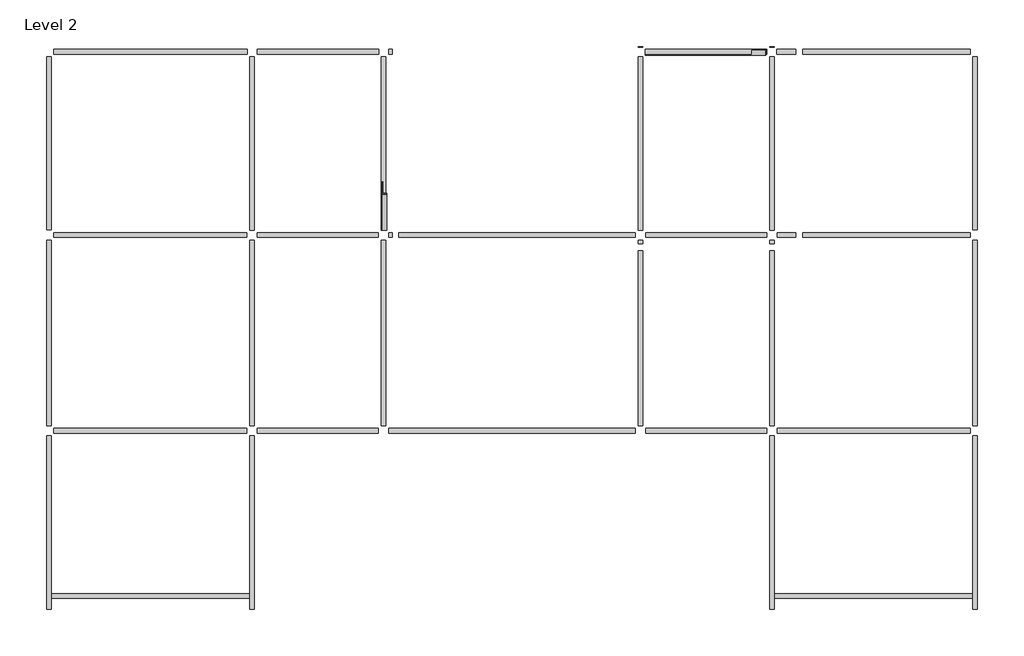
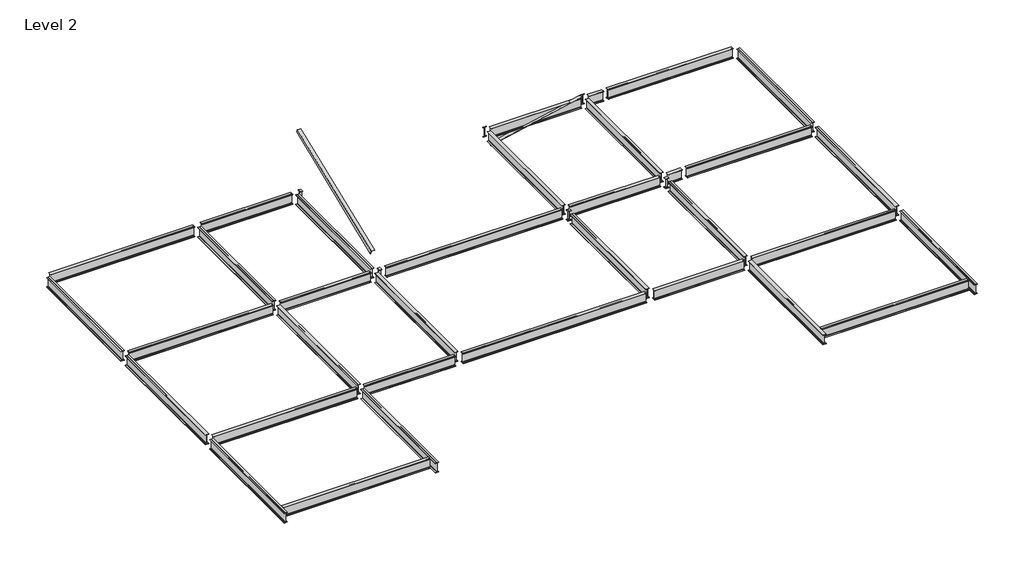
# One storey: 40 beams, 2 members.
"""IFC4 building model written with IfcOpenShell, lengths in millimetres."""

import ifcopenshell
import ifcopenshell.guid

model = None  # the IFC model being written
_history = None  # IfcOwnerHistory: only IFC2X3 demands one
_inside = {}  # id of a spatial element -> (the spatial element, [elements in it])
_under = {}  # id of a project, library or spatial element -> (it, [spatial elements below it])
_declared = {}  # id of a project -> (the project, [libraries it declares])
_typed = {}  # id of a type object -> (the type object, [elements of that type])
_made_of = {}  # id of a material, layer set ... -> (it, [elements and type objects made of it])


def new_model(schema):
    """Start an empty IFC model of exactly this schema.

    Asked for "IFC4X3", IfcOpenShell would pick the latest addendum, in which some entities
    have other attributes; the version numbers below select the first issue.
    IFC2X3 requires an IfcOwnerHistory on every rooted entity: one is made here for all.
    """
    global model, _history
    if schema == "IFC4X3":
        model = ifcopenshell.file(schema_version=(4, 3, 0, 0))
    else:
        model = ifcopenshell.file(schema=schema)
    _inside.clear()
    _under.clear()
    _declared.clear()
    _typed.clear()
    _made_of.clear()
    _history = None
    if model.schema == "IFC2X3":
        org = make("IfcOrganization", Name="unknown")
        user = make(
            "IfcPersonAndOrganization",
            ThePerson=make("IfcPerson", FamilyName="unknown"),
            TheOrganization=org,
        )
        app = make(
            "IfcApplication",
            ApplicationDeveloper=org,
            Version="unknown",
            ApplicationFullName="unknown",
            ApplicationIdentifier="unknown",
        )
        _history = make(
            "IfcOwnerHistory",
            OwningUser=user,
            OwningApplication=app,
            ChangeAction="ADDED",
            CreationDate=0,
        )
    return model


def make(cls, **values):
    """One entity of the class cls with the attributes given. An attribute that is None is left unset."""
    return model.create_entity(
        cls, **{name: value for name, value in values.items() if value is not None}
    )


def rooted(cls, **values):
    """An entity with a GlobalId (a new one), such as an element, a storey or a relation."""
    return make(cls, GlobalId=ifcopenshell.guid.new(), OwnerHistory=_history, **values)


def si_unit(unit_type, name, prefix=None):
    """IfcSIUnit, for example si_unit("LENGTHUNIT", "METRE", prefix="MILLI")."""
    return make("IfcSIUnit", UnitType=unit_type, Prefix=prefix, Name=name)


def assignment(units):
    """IfcUnitAssignment: the units of a project."""
    return None if units is None else make("IfcUnitAssignment", Units=units)


def point(xyz):
    """IfcCartesianPoint."""
    return None if xyz is None else make("IfcCartesianPoint", Coordinates=xyz)


def direction(xyz):
    """IfcDirection."""
    return None if xyz is None else make("IfcDirection", DirectionRatios=xyz)


def frame(location, z_axis=None, x_axis=None):
    """IfcAxis2Placement3D, a coordinate frame: its origin and axes. An axis left out is left unset."""
    return make(
        "IfcAxis2Placement3D",
        Location=point(location),
        Axis=direction(z_axis),
        RefDirection=direction(x_axis),
    )


def frame_2d(location, x_axis=None):
    """IfcAxis2Placement2D, a coordinate frame in the plane: its origin and x axis."""
    return make(
        "IfcAxis2Placement2D", Location=point(location), RefDirection=direction(x_axis)
    )


def origin():
    """The frame at (0, 0, 0) with its axes left unset."""
    return frame((0.0, 0.0, 0.0))


def place(relative_to, where):
    """IfcLocalPlacement: puts the frame where relative to a parent placement (None: the world)."""
    return make(
        "IfcLocalPlacement", PlacementRelTo=relative_to, RelativePlacement=where
    )


def context(
    kind, dimensions, precision=None, world=None, true_north=None, identifier=None
):
    """IfcGeometricRepresentationContext, for example the 3D "Model" context."""
    return make(
        "IfcGeometricRepresentationContext",
        ContextIdentifier=identifier,
        ContextType=kind,
        CoordinateSpaceDimension=dimensions,
        Precision=precision,
        WorldCoordinateSystem=world,
        TrueNorth=true_north,
    )


def project(units=None, contexts=None):
    """IfcProject with its units and contexts."""
    return rooted(
        "IfcProject",
        Name="project",
        RepresentationContexts=contexts,
        UnitsInContext=assignment(units),
    )


def spatial(cls, under=None, at=None, **own):
    """A site, building, storey or space (cls), placed at a placement, below another one or the project."""
    s = rooted(cls, ObjectPlacement=at, **own)
    if under is not None:
        _under.setdefault(under.id(), (under, []))[1].append(s)
    return s


def polyline(points):
    """IfcPolyline through the points."""
    return make("IfcPolyline", Points=[point(p) for p in points])


def circle_curve(where, radius):
    """IfcCircle in the frame where."""
    return make("IfcCircle", Position=where, Radius=radius)


def trimmed(basis, trim1, trim2, sense, master):
    """IfcTrimmedCurve: the piece of a basis curve between two trims."""
    return make(
        "IfcTrimmedCurve",
        BasisCurve=basis,
        Trim1=trim1,
        Trim2=trim2,
        SenseAgreement=sense,
        MasterRepresentation=master,
    )


def segment(curve, same_sense, transition):
    """IfcCompositeCurveSegment."""
    return make(
        "IfcCompositeCurveSegment",
        Transition=transition,
        SameSense=same_sense,
        ParentCurve=curve,
    )


def composite_curve(segments, self_intersect=None):
    """IfcCompositeCurve: segments joined end to end."""
    return make("IfcCompositeCurve", Segments=segments, SelfIntersect=self_intersect)


def outline(outer, holes=None, kind="AREA"):
    """IfcArbitraryClosedProfileDef: a profile drawn as a closed curve; with holes, ...WithVoids."""
    if holes is None:
        return make("IfcArbitraryClosedProfileDef", ProfileType=kind, OuterCurve=outer)
    return make(
        "IfcArbitraryProfileDefWithVoids",
        ProfileType=kind,
        OuterCurve=outer,
        InnerCurves=holes,
    )


def extrude(swept, where, along, depth):
    """IfcExtrudedAreaSolid: the profile swept, set in the frame where, extruded along a direction by depth."""
    return make(
        "IfcExtrudedAreaSolid",
        SweptArea=swept,
        Position=where,
        ExtrudedDirection=direction(along),
        Depth=depth,
    )


def shape(context_of_items, identifier, shape_type, items):
    """IfcShapeRepresentation: the items that make up one representation, for example the "Body"."""
    return make(
        "IfcShapeRepresentation",
        ContextOfItems=context_of_items,
        RepresentationIdentifier=identifier,
        RepresentationType=shape_type,
        Items=items,
    )


def source(mapping_origin, context_of_items, identifier, shape_type, items):
    """IfcRepresentationMap: a shape defined once, which mapped items show again and again."""
    return make(
        "IfcRepresentationMap",
        MappingOrigin=mapping_origin,
        MappedRepresentation=shape(context_of_items, identifier, shape_type, items),
    )


def transform(
    local_origin,
    x_axis=None,
    y_axis=None,
    z_axis=None,
    scale=None,
    scale2=None,
    scale3=None,
    uniform=True,
):
    """IfcCartesianTransformationOperator3D, or its non-uniform kind. x_axis, y_axis, z_axis: its Axis1, 2, 3."""
    if uniform:
        return make(
            "IfcCartesianTransformationOperator3D",
            Axis1=direction(x_axis),
            Axis2=direction(y_axis),
            LocalOrigin=point(local_origin),
            Scale=scale,
            Axis3=direction(z_axis),
        )
    return make(
        "IfcCartesianTransformationOperator3DnonUniform",
        Axis1=direction(x_axis),
        Axis2=direction(y_axis),
        LocalOrigin=point(local_origin),
        Scale=scale,
        Axis3=direction(z_axis),
        Scale2=scale2,
        Scale3=scale3,
    )


def mapped(mapping_source, mapping_target):
    """IfcMappedItem: shows the shape of a source again, moved by a transform."""
    return make(
        "IfcMappedItem", MappingSource=mapping_source, MappingTarget=mapping_target
    )


def made_of(thing, what):
    """Note that an element or type object is made of a material, layer set ...; save() writes the relation."""
    if what is not None:
        _made_of.setdefault(what.id(), (what, []))[1].append(thing)
    return thing


def element(
    cls,
    number,
    at=None,
    inside=None,
    cuts=None,
    type_object=None,
    material=None,
    context=None,
    identifier="Body",
    shape_type=None,
    held_by="IfcProductDefinitionShape",
    body=None,
    shapes=None,
    **own,
):
    """One element of the class cls, such as IfcWall. Its Tag is "e" and its number.

    at: its placement. inside: the storey or other place that contains it. cuts: it is an
    opening in that element (IfcRelVoidsElement). A single representation is given by context,
    identifier, shape_type and body (its items); several are given by shapes. held_by: the class
    of the entity that holds the representations. save() writes the other relations.
    """
    e = rooted(cls, Tag="e%d" % number, ObjectPlacement=at, **own)
    if body is not None:
        shapes = [shape(context, identifier, shape_type, body)]
    if shapes is not None:
        e.Representation = make(held_by, Representations=shapes)
    if inside is not None:
        _inside.setdefault(inside.id(), (inside, []))[1].append(e)
    if cuts is not None:
        rooted(
            "IfcRelVoidsElement", RelatingBuildingElement=cuts, RelatedOpeningElement=e
        )
    if type_object is not None:
        _typed.setdefault(type_object.id(), (type_object, []))[1].append(e)
    return made_of(e, material)


def aggregate(whole, parts):
    """IfcRelAggregates: a whole, such as a stair, and the parts it consists of."""
    return rooted("IfcRelAggregates", RelatingObject=whole, RelatedObjects=parts)


def save(model, path):
    """Write the relations noted so far, then the file.

    IfcRelAggregates (storeys below a building ...), IfcRelContainedInSpatialStructure (elements
    in a storey), IfcRelDefinesByType, IfcRelAssociatesMaterial and IfcRelDeclares: one each for
    every whole, place, type object, material and project.
    """
    for whole, parts in _under.values():
        aggregate(whole, parts)
    for where, things in _inside.values():
        rooted(
            "IfcRelContainedInSpatialStructure",
            RelatedElements=things,
            RelatingStructure=where,
        )
    for kind, things in _typed.values():
        rooted("IfcRelDefinesByType", RelatedObjects=things, RelatingType=kind)
    for what, things in _made_of.values():
        rooted("IfcRelAssociatesMaterial", RelatedObjects=things, RelatingMaterial=what)
    for by, libraries in _declared.values():
        rooted("IfcRelDeclares", RelatingContext=by, RelatedDefinitions=libraries)
    model.write(path)


def w_wide_flange2_w18x40_53786035(model_context):
    return source(origin(), model_context, "Body", "SweptSolid", [
        extrude(outline(composite_curve([segment(polyline([(76.454, -213.995), (76.454, -227.33), (-76.454, -227.33), (-76.454, -213.995), (-20.828, -213.995)]), True, "CONTINUOUS"), segment(trimmed(circle_curve(frame_2d((-20.828, -197.1675)), 16.8275), [point((-20.828, -213.995))], [point((-4.0005, -197.1675))], True, "CARTESIAN"), True, "CONTINUOUS"), segment(polyline([(-4.0005, -197.1675), (-4.0005, 197.1675)]), True, "CONTINUOUS"), segment(trimmed(circle_curve(frame_2d((-20.828, 197.1675)), 16.8275), [point((-4.0005, 197.1675))], [point((-20.828, 213.995))], True, "CARTESIAN"), True, "CONTINUOUS"), segment(polyline([(-20.828, 213.995), (-76.454, 213.995), (-76.454, 227.33), (76.454, 227.33), (76.454, 213.995), (20.828, 213.995)]), True, "CONTINUOUS"), segment(trimmed(circle_curve(frame_2d((20.828, 197.1675)), 16.8275), [point((20.828, 213.995))], [point((4.0005, 197.1675))], True, "CARTESIAN"), True, "CONTINUOUS"), segment(polyline([(4.0005, 197.1675), (4.0005, -197.1675)]), True, "CONTINUOUS"), segment(trimmed(circle_curve(frame_2d((20.828, -197.1675)), 16.8275), [point((4.0005, -197.1675))], [point((20.828, -213.995))], True, "CARTESIAN"), True, "CONTINUOUS"), segment(polyline([(20.828, -213.995), (76.454, -213.995)]), True, "CONTINUOUS")], self_intersect=False)), frame((-3289.046, 0.0, 0.0), z_axis=(1.0, 0.0, 0.0), x_axis=(0.0, 1.0, 0.0)), (0.0, 0.0, 1.0), 6578.092),
    ])


def w_wide_flange2_w18x40_11743c99(model_context):
    return source(origin(), model_context, "Body", "SweptSolid", [
        extrude(outline(composite_curve([segment(polyline([(76.454, -213.995), (76.454, -227.33), (-76.454, -227.33), (-76.454, -213.995), (-20.828, -213.995)]), True, "CONTINUOUS"), segment(trimmed(circle_curve(frame_2d((-20.828, -197.1675)), 16.8275), [point((-20.828, -213.995))], [point((-4.0005, -197.1675))], True, "CARTESIAN"), True, "CONTINUOUS"), segment(polyline([(-4.0005, -197.1675), (-4.0005, 197.1675)]), True, "CONTINUOUS"), segment(trimmed(circle_curve(frame_2d((-20.828, 197.1675)), 16.8275), [point((-4.0005, 197.1675))], [point((-20.828, 213.995))], True, "CARTESIAN"), True, "CONTINUOUS"), segment(polyline([(-20.828, 213.995), (-76.454, 213.995), (-76.454, 227.33), (76.454, 227.33), (76.454, 213.995), (20.828, 213.995)]), True, "CONTINUOUS"), segment(trimmed(circle_curve(frame_2d((20.828, 197.1675)), 16.8275), [point((20.828, 213.995))], [point((4.0005, 197.1675))], True, "CARTESIAN"), True, "CONTINUOUS"), segment(polyline([(4.0005, 197.1675), (4.0005, -197.1675)]), True, "CONTINUOUS"), segment(trimmed(circle_curve(frame_2d((20.828, -197.1675)), 16.8275), [point((4.0005, -197.1675))], [point((20.828, -213.995))], True, "CARTESIAN"), True, "CONTINUOUS"), segment(polyline([(20.828, -213.995), (76.454, -213.995)]), True, "CONTINUOUS")], self_intersect=False)), frame((-3211.5125, 0.0, 0.0), z_axis=(1.0, 0.0, 0.0), x_axis=(0.0, 1.0, 0.0)), (0.0, 0.0, 1.0), 6423.025),
    ])


def w_wide_flange2_w18x40_35389f5a(model_context):
    return source(origin(), model_context, "Body", "SweptSolid", [
        extrude(outline(composite_curve([segment(polyline([(76.454, -213.995), (76.454, -227.33), (-76.454, -227.33), (-76.454, -213.995), (-20.828, -213.995)]), True, "CONTINUOUS"), segment(trimmed(circle_curve(frame_2d((-20.828, -197.1675)), 16.8275), [point((-20.828, -213.995))], [point((-4.0005, -197.1675))], True, "CARTESIAN"), True, "CONTINUOUS"), segment(polyline([(-4.0005, -197.1675), (-4.0005, 197.1675)]), True, "CONTINUOUS"), segment(trimmed(circle_curve(frame_2d((-20.828, 197.1675)), 16.8275), [point((-4.0005, 197.1675))], [point((-20.828, 213.995))], True, "CARTESIAN"), True, "CONTINUOUS"), segment(polyline([(-20.828, 213.995), (-76.454, 213.995), (-76.454, 227.33), (76.454, 227.33), (76.454, 213.995), (20.828, 213.995)]), True, "CONTINUOUS"), segment(trimmed(circle_curve(frame_2d((20.828, 197.1675)), 16.8275), [point((20.828, 213.995))], [point((4.0005, 197.1675))], True, "CARTESIAN"), True, "CONTINUOUS"), segment(polyline([(4.0005, 197.1675), (4.0005, -197.1675)]), True, "CONTINUOUS"), segment(trimmed(circle_curve(frame_2d((20.828, -197.1675)), 16.8275), [point((4.0005, -197.1675))], [point((20.828, -213.995))], True, "CARTESIAN"), True, "CONTINUOUS"), segment(polyline([(20.828, -213.995), (76.454, -213.995)]), True, "CONTINUOUS")], self_intersect=False)), frame((-2017.7125, 0.0, 0.0), z_axis=(1.0, 0.0, 0.0), x_axis=(0.0, 1.0, 0.0)), (0.0, 0.0, 1.0), 4035.425),
    ])


def w_wide_flange2_w18x40_cea889e1(model_context):
    return source(origin(), model_context, "Body", "SweptSolid", [
        extrude(outline(composite_curve([segment(polyline([(76.454, -213.995), (76.454, -227.33), (-76.454, -227.33), (-76.454, -213.995), (-20.828, -213.995)]), True, "CONTINUOUS"), segment(trimmed(circle_curve(frame_2d((-20.828, -197.1675)), 16.8275), [point((-20.828, -213.995))], [point((-4.0005, -197.1675))], True, "CARTESIAN"), True, "CONTINUOUS"), segment(polyline([(-4.0005, -197.1675), (-4.0005, 197.1675)]), True, "CONTINUOUS"), segment(trimmed(circle_curve(frame_2d((-20.828, 197.1675)), 16.8275), [point((-4.0005, 197.1675))], [point((-20.828, 213.995))], True, "CARTESIAN"), True, "CONTINUOUS"), segment(polyline([(-20.828, 213.995), (-76.454, 213.995), (-76.454, 227.33), (76.454, 227.33), (76.454, 213.995), (20.828, 213.995)]), True, "CONTINUOUS"), segment(trimmed(circle_curve(frame_2d((20.828, 197.1675)), 16.8275), [point((20.828, 213.995))], [point((4.0005, 197.1675))], True, "CARTESIAN"), True, "CONTINUOUS"), segment(polyline([(4.0005, 197.1675), (4.0005, -197.1675)]), True, "CONTINUOUS"), segment(trimmed(circle_curve(frame_2d((20.828, -197.1675)), 16.8275), [point((4.0005, -197.1675))], [point((20.828, -213.995))], True, "CARTESIAN"), True, "CONTINUOUS"), segment(polyline([(20.828, -213.995), (76.454, -213.995)]), True, "CONTINUOUS")], self_intersect=False)), frame((-3211.5125, 0.0, 0.0), z_axis=(1.0, 0.0, 0.0), x_axis=(0.0, 1.0, 0.0)), (0.0, 0.0, 1.0), 6417.865625),
    ])


def w_wide_flange2_w18x40_962a7e4b(model_context):
    return source(origin(), model_context, "Body", "SweptSolid", [
        extrude(outline(composite_curve([segment(polyline([(76.454, -213.995), (76.454, -227.33), (-76.454, -227.33), (-76.454, -213.995), (-20.828, -213.995)]), True, "CONTINUOUS"), segment(trimmed(circle_curve(frame_2d((-20.828, -197.1675)), 16.8275), [point((-20.828, -213.995))], [point((-4.0005, -197.1675))], True, "CARTESIAN"), True, "CONTINUOUS"), segment(polyline([(-4.0005, -197.1675), (-4.0005, 197.1675)]), True, "CONTINUOUS"), segment(trimmed(circle_curve(frame_2d((-20.828, 197.1675)), 16.8275), [point((-4.0005, 197.1675))], [point((-20.828, 213.995))], True, "CARTESIAN"), True, "CONTINUOUS"), segment(polyline([(-20.828, 213.995), (-76.454, 213.995), (-76.454, 227.33), (76.454, 227.33), (76.454, 213.995), (20.828, 213.995)]), True, "CONTINUOUS"), segment(trimmed(circle_curve(frame_2d((20.828, 197.1675)), 16.8275), [point((20.828, 213.995))], [point((4.0005, 197.1675))], True, "CARTESIAN"), True, "CONTINUOUS"), segment(polyline([(4.0005, 197.1675), (4.0005, -197.1675)]), True, "CONTINUOUS"), segment(trimmed(circle_curve(frame_2d((20.828, -197.1675)), 16.8275), [point((4.0005, -197.1675))], [point((20.828, -213.995))], True, "CARTESIAN"), True, "CONTINUOUS"), segment(polyline([(20.828, -213.995), (76.454, -213.995)]), True, "CONTINUOUS")], self_intersect=False)), frame((-2012.553125, 0.0, 0.0), z_axis=(1.0, 0.0, 0.0), x_axis=(0.0, 1.0, 0.0)), (0.0, 0.0, 1.0), 4025.10625),
    ])


def w_wide_flange2_w18x40_41391f11(model_context):
    return source(origin(), model_context, "Body", "SweptSolid", [
        extrude(outline(composite_curve([segment(polyline([(76.454, -213.995), (76.454, -227.33), (-76.454, -227.33), (-76.454, -213.995), (-20.828, -213.995)]), True, "CONTINUOUS"), segment(trimmed(circle_curve(frame_2d((-20.828, -197.1675)), 16.8275), [point((-20.828, -213.995))], [point((-4.0005, -197.1675))], True, "CARTESIAN"), True, "CONTINUOUS"), segment(polyline([(-4.0005, -197.1675), (-4.0005, 197.1675)]), True, "CONTINUOUS"), segment(trimmed(circle_curve(frame_2d((-20.828, 197.1675)), 16.8275), [point((-4.0005, 197.1675))], [point((-20.828, 213.995))], True, "CARTESIAN"), True, "CONTINUOUS"), segment(polyline([(-20.828, 213.995), (-76.454, 213.995), (-76.454, 227.33), (76.454, 227.33), (76.454, 213.995), (20.828, 213.995)]), True, "CONTINUOUS"), segment(trimmed(circle_curve(frame_2d((20.828, 197.1675)), 16.8275), [point((20.828, 213.995))], [point((4.0005, 197.1675))], True, "CARTESIAN"), True, "CONTINUOUS"), segment(polyline([(4.0005, 197.1675), (4.0005, -197.1675)]), True, "CONTINUOUS"), segment(trimmed(circle_curve(frame_2d((20.828, -197.1675)), 16.8275), [point((4.0005, -197.1675))], [point((20.828, -213.995))], True, "CARTESIAN"), True, "CONTINUOUS"), segment(polyline([(20.828, -213.995), (76.454, -213.995)]), True, "CONTINUOUS")], self_intersect=False)), frame((-4095.353125, 0.0, 0.0), z_axis=(1.0, 0.0, 0.0), x_axis=(0.0, 1.0, 0.0)), (0.0, 0.0, 1.0), 8190.70625),
    ])


def w_wide_flange2_w18x40_1ff26780(model_context):
    return source(origin(), model_context, "Body", "SweptSolid", [
        extrude(outline(composite_curve([segment(polyline([(76.454, -213.995), (76.454, -227.33), (-76.454, -227.33), (-76.454, -213.995), (-20.828, -213.995)]), True, "CONTINUOUS"), segment(trimmed(circle_curve(frame_2d((-20.828, -197.1675)), 16.8275), [point((-20.828, -213.995))], [point((-4.0005, -197.1675))], True, "CARTESIAN"), True, "CONTINUOUS"), segment(polyline([(-4.0005, -197.1675), (-4.0005, 197.1675)]), True, "CONTINUOUS"), segment(trimmed(circle_curve(frame_2d((-20.828, 197.1675)), 16.8275), [point((-4.0005, 197.1675))], [point((-20.828, 213.995))], True, "CARTESIAN"), True, "CONTINUOUS"), segment(polyline([(-20.828, 213.995), (-76.454, 213.995), (-76.454, 227.33), (76.454, 227.33), (76.454, 213.995), (20.828, 213.995)]), True, "CONTINUOUS"), segment(trimmed(circle_curve(frame_2d((20.828, 197.1675)), 16.8275), [point((20.828, 213.995))], [point((4.0005, 197.1675))], True, "CARTESIAN"), True, "CONTINUOUS"), segment(polyline([(4.0005, 197.1675), (4.0005, -197.1675)]), True, "CONTINUOUS"), segment(trimmed(circle_curve(frame_2d((20.828, -197.1675)), 16.8275), [point((4.0005, -197.1675))], [point((20.828, -213.995))], True, "CARTESIAN"), True, "CONTINUOUS"), segment(polyline([(20.828, -213.995), (76.454, -213.995)]), True, "CONTINUOUS")], self_intersect=False)), frame((-3206.353125, 0.0, 0.0), z_axis=(1.0, 0.0, 0.0), x_axis=(0.0, 1.0, 0.0)), (0.0, 0.0, 1.0), 6417.865625),
    ])


def w_wide_flange2_w18x40_a80abbf0(model_context):
    return source(origin(), model_context, "Body", "SweptSolid", [
        extrude(outline(composite_curve([segment(polyline([(76.454, -213.995), (76.454, -227.33), (-76.454, -227.33), (-76.454, -213.995), (-20.828, -213.995)]), True, "CONTINUOUS"), segment(trimmed(circle_curve(frame_2d((-20.828, -197.1675)), 16.8275), [point((-20.828, -213.995))], [point((-4.0005, -197.1675))], True, "CARTESIAN"), True, "CONTINUOUS"), segment(polyline([(-4.0005, -197.1675), (-4.0005, 197.1675)]), True, "CONTINUOUS"), segment(trimmed(circle_curve(frame_2d((-20.828, 197.1675)), 16.8275), [point((-4.0005, 197.1675))], [point((-20.828, 213.995))], True, "CARTESIAN"), True, "CONTINUOUS"), segment(polyline([(-20.828, 213.995), (-76.454, 213.995), (-76.454, 227.33), (76.454, 227.33), (76.454, 213.995), (20.828, 213.995)]), True, "CONTINUOUS"), segment(trimmed(circle_curve(frame_2d((20.828, 197.1675)), 16.8275), [point((20.828, 213.995))], [point((4.0005, 197.1675))], True, "CARTESIAN"), True, "CONTINUOUS"), segment(polyline([(4.0005, 197.1675), (4.0005, -197.1675)]), True, "CONTINUOUS"), segment(trimmed(circle_curve(frame_2d((20.828, -197.1675)), 16.8275), [point((4.0005, -197.1675))], [point((20.828, -213.995))], True, "CARTESIAN"), True, "CONTINUOUS"), segment(polyline([(20.828, -213.995), (76.454, -213.995)]), True, "CONTINUOUS")], self_intersect=False)), frame((-2876.153125, 0.0, 0.0), z_axis=(1.0, 0.0, 0.0), x_axis=(0.0, 1.0, 0.0)), (0.0, 0.0, 1.0), 5752.30625),
    ])


def w_wide_flange2_w18x40_30b59f7b(model_context):
    return source(origin(), model_context, "Body", "SweptSolid", [
        extrude(outline(composite_curve([segment(polyline([(76.454, -213.995), (76.454, -227.33), (-76.454, -227.33), (-76.454, -213.995), (-20.828, -213.995)]), True, "CONTINUOUS"), segment(trimmed(circle_curve(frame_2d((-20.828, -197.1675)), 16.8275), [point((-20.828, -213.995))], [point((-4.0005, -197.1675))], True, "CARTESIAN"), True, "CONTINUOUS"), segment(polyline([(-4.0005, -197.1675), (-4.0005, 197.1675)]), True, "CONTINUOUS"), segment(trimmed(circle_curve(frame_2d((-20.828, 197.1675)), 16.8275), [point((-4.0005, 197.1675))], [point((-20.828, 213.995))], True, "CARTESIAN"), True, "CONTINUOUS"), segment(polyline([(-20.828, 213.995), (-76.454, 213.995), (-76.454, 227.33), (76.454, 227.33), (76.454, 213.995), (20.828, 213.995)]), True, "CONTINUOUS"), segment(trimmed(circle_curve(frame_2d((20.828, 197.1675)), 16.8275), [point((20.828, 213.995))], [point((4.0005, 197.1675))], True, "CARTESIAN"), True, "CONTINUOUS"), segment(polyline([(4.0005, 197.1675), (4.0005, -197.1675)]), True, "CONTINUOUS"), segment(trimmed(circle_curve(frame_2d((20.828, -197.1675)), 16.8275), [point((4.0005, -197.1675))], [point((20.828, -213.995))], True, "CARTESIAN"), True, "CONTINUOUS"), segment(polyline([(20.828, -213.995), (76.454, -213.995)]), True, "CONTINUOUS")], self_intersect=False)), frame((-3079.353125, 0.0, 0.0), z_axis=(1.0, 0.0, 0.0), x_axis=(0.0, 1.0, 0.0)), (0.0, 0.0, 1.0), 6158.70625),
    ])


def w_wide_flange2_w18x40_ca46fc5e(model_context):
    return source(origin(), model_context, "Body", "SweptSolid", [
        extrude(outline(composite_curve([segment(polyline([(76.454, -213.995), (76.454, -227.33), (-76.454, -227.33), (-76.454, -213.995), (-20.828, -213.995)]), True, "CONTINUOUS"), segment(trimmed(circle_curve(frame_2d((-20.828, -197.1675)), 16.8275), [point((-20.828, -213.995))], [point((-4.0005, -197.1675))], True, "CARTESIAN"), True, "CONTINUOUS"), segment(polyline([(-4.0005, -197.1675), (-4.0005, 197.1675)]), True, "CONTINUOUS"), segment(trimmed(circle_curve(frame_2d((-20.828, 197.1675)), 16.8275), [point((-4.0005, 197.1675))], [point((-20.828, 213.995))], True, "CARTESIAN"), True, "CONTINUOUS"), segment(polyline([(-20.828, 213.995), (-76.454, 213.995), (-76.454, 227.33), (76.454, 227.33), (76.454, 213.995), (20.828, 213.995)]), True, "CONTINUOUS"), segment(trimmed(circle_curve(frame_2d((20.828, 197.1675)), 16.8275), [point((20.828, 213.995))], [point((4.0005, 197.1675))], True, "CARTESIAN"), True, "CONTINUOUS"), segment(polyline([(4.0005, 197.1675), (4.0005, -197.1675)]), True, "CONTINUOUS"), segment(trimmed(circle_curve(frame_2d((20.828, -197.1675)), 16.8275), [point((4.0005, -197.1675))], [point((20.828, -213.995))], True, "CARTESIAN"), True, "CONTINUOUS"), segment(polyline([(20.828, -213.995), (76.454, -213.995)]), True, "CONTINUOUS")], self_intersect=False)), frame((-2876.153125, 0.0, 0.0), z_axis=(1.0, 0.0, 0.0), x_axis=(0.0, 1.0, 0.0)), (0.0, 0.0, 1.0), 5757.465625),
    ])


def w_wide_flange2_w18x40_9a74fa6d(model_context):
    return source(origin(), model_context, "Body", "SweptSolid", [
        extrude(outline(composite_curve([segment(polyline([(76.454, -213.995), (76.454, -227.33), (-76.454, -227.33), (-76.454, -213.995), (-20.828, -213.995)]), True, "CONTINUOUS"), segment(trimmed(circle_curve(frame_2d((-20.828, -197.1675)), 16.8275), [point((-20.828, -213.995))], [point((-4.0005, -197.1675))], True, "CARTESIAN"), True, "CONTINUOUS"), segment(polyline([(-4.0005, -197.1675), (-4.0005, 197.1675)]), True, "CONTINUOUS"), segment(trimmed(circle_curve(frame_2d((-20.828, 197.1675)), 16.8275), [point((-4.0005, 197.1675))], [point((-20.828, 213.995))], True, "CARTESIAN"), True, "CONTINUOUS"), segment(polyline([(-20.828, 213.995), (-76.454, 213.995), (-76.454, 227.33), (76.454, 227.33), (76.454, 213.995), (20.828, 213.995)]), True, "CONTINUOUS"), segment(trimmed(circle_curve(frame_2d((20.828, 197.1675)), 16.8275), [point((20.828, 213.995))], [point((4.0005, 197.1675))], True, "CARTESIAN"), True, "CONTINUOUS"), segment(polyline([(4.0005, 197.1675), (4.0005, -197.1675)]), True, "CONTINUOUS"), segment(trimmed(circle_curve(frame_2d((20.828, -197.1675)), 16.8275), [point((4.0005, -197.1675))], [point((20.828, -213.995))], True, "CARTESIAN"), True, "CONTINUOUS"), segment(polyline([(20.828, -213.995), (76.454, -213.995)]), True, "CONTINUOUS")], self_intersect=False)), frame((-3084.5125, 0.0, 0.0), z_axis=(1.0, 0.0, 0.0), x_axis=(0.0, 1.0, 0.0)), (0.0, 0.0, 1.0), 6169.025),
    ])


def w_wide_flange2_w18x40_66fddd83(model_context):
    return source(origin(), model_context, "Body", "SweptSolid", [
        extrude(outline(composite_curve([segment(polyline([(76.454, -213.995), (76.454, -227.33), (-76.454, -227.33), (-76.454, -213.995), (-20.828, -213.995)]), True, "CONTINUOUS"), segment(trimmed(circle_curve(frame_2d((-20.828, -197.1675)), 16.8275), [point((-20.828, -213.995))], [point((-4.0005, -197.1675))], True, "CARTESIAN"), True, "CONTINUOUS"), segment(polyline([(-4.0005, -197.1675), (-4.0005, 197.1675)]), True, "CONTINUOUS"), segment(trimmed(circle_curve(frame_2d((-20.828, 197.1675)), 16.8275), [point((-4.0005, 197.1675))], [point((-20.828, 213.995))], True, "CARTESIAN"), True, "CONTINUOUS"), segment(polyline([(-20.828, 213.995), (-76.454, 213.995), (-76.454, 227.33), (76.454, 227.33), (76.454, 213.995), (20.828, 213.995)]), True, "CONTINUOUS"), segment(trimmed(circle_curve(frame_2d((20.828, 197.1675)), 16.8275), [point((20.828, 213.995))], [point((4.0005, 197.1675))], True, "CARTESIAN"), True, "CONTINUOUS"), segment(polyline([(4.0005, 197.1675), (4.0005, -197.1675)]), True, "CONTINUOUS"), segment(trimmed(circle_curve(frame_2d((20.828, -197.1675)), 16.8275), [point((4.0005, -197.1675))], [point((20.828, -213.995))], True, "CARTESIAN"), True, "CONTINUOUS"), segment(polyline([(20.828, -213.995), (76.454, -213.995)]), True, "CONTINUOUS")], self_intersect=False)), frame((-2881.3125, 0.0, 0.0), z_axis=(1.0, 0.0, 0.0), x_axis=(0.0, 1.0, 0.0)), (0.0, 0.0, 1.0), 5757.465625),
    ])


def w_wide_flange2_w18x40_cd45667b(model_context):
    return source(origin(), model_context, "Body", "SweptSolid", [
        extrude(outline(composite_curve([segment(polyline([(-76.454, -213.995), (-20.828, -213.995)]), True, "CONTINUOUS"), segment(trimmed(circle_curve(frame_2d((-20.828, -197.1675)), 16.8275), [point((-20.828, -213.995))], [point((-4.0005, -197.1675))], True, "CARTESIAN"), True, "CONTINUOUS"), segment(polyline([(-4.0005, -197.1675), (-4.0005, 197.1675)]), True, "CONTINUOUS"), segment(trimmed(circle_curve(frame_2d((-20.828, 197.1675)), 16.8275), [point((-4.0005, 197.1675))], [point((-20.828, 213.995))], True, "CARTESIAN"), True, "CONTINUOUS"), segment(polyline([(-20.828, 213.995), (-76.454, 213.995), (-76.454, 227.33), (76.454, 227.33), (76.454, 213.995), (20.828, 213.995)]), True, "CONTINUOUS"), segment(trimmed(circle_curve(frame_2d((20.828, 197.1675)), 16.8275), [point((20.828, 213.995))], [point((4.0005, 197.1675))], True, "CARTESIAN"), True, "CONTINUOUS"), segment(polyline([(4.0005, 197.1675), (4.0005, -197.1675)]), True, "CONTINUOUS"), segment(trimmed(circle_curve(frame_2d((20.828, -197.1675)), 16.8275), [point((4.0005, -197.1675))], [point((20.828, -213.995))], True, "CARTESIAN"), True, "CONTINUOUS"), segment(polyline([(20.828, -213.995), (76.454, -213.995), (76.454, -227.33), (-76.454, -227.33), (-76.454, -213.995)]), True, "CONTINUOUS")], self_intersect=False)), frame((19.84375, 0.0, 0.0), z_axis=(1.0, 0.0, 0.0), x_axis=(0.0, 1.0, 0.0)), (0.0, 0.0, 1.0), 22.621875),
    ])


def w_wide_flange2_w18x40_42c25f9a(model_context):
    return source(origin(), model_context, "Body", "SweptSolid", [
        extrude(outline(composite_curve([segment(polyline([(76.454, -213.995), (76.454, -227.33), (-76.454, -227.33), (-76.454, -213.995), (-20.828, -213.995)]), True, "CONTINUOUS"), segment(trimmed(circle_curve(frame_2d((-20.828, -197.1675)), 16.8275), [point((-20.828, -213.995))], [point((-4.0005, -197.1675))], True, "CARTESIAN"), True, "CONTINUOUS"), segment(polyline([(-4.0005, -197.1675), (-4.0005, 197.1675)]), True, "CONTINUOUS"), segment(trimmed(circle_curve(frame_2d((-20.828, 197.1675)), 16.8275), [point((-4.0005, 197.1675))], [point((-20.828, 213.995))], True, "CARTESIAN"), True, "CONTINUOUS"), segment(polyline([(-20.828, 213.995), (-76.454, 213.995), (-76.454, 227.33), (76.454, 227.33), (76.454, 213.995), (20.828, 213.995)]), True, "CONTINUOUS"), segment(trimmed(circle_curve(frame_2d((20.828, 197.1675)), 16.8275), [point((20.828, 213.995))], [point((4.0005, 197.1675))], True, "CARTESIAN"), True, "CONTINUOUS"), segment(polyline([(4.0005, 197.1675), (4.0005, -197.1675)]), True, "CONTINUOUS"), segment(trimmed(circle_curve(frame_2d((20.828, -197.1675)), 16.8275), [point((4.0005, -197.1675))], [point((20.828, -213.995))], True, "CARTESIAN"), True, "CONTINUOUS"), segment(polyline([(20.828, -213.995), (76.454, -213.995)]), True, "CONTINUOUS")], self_intersect=False)), frame((-2756.69375, 0.0, 0.0), z_axis=(1.0, 0.0, 0.0), x_axis=(0.0, 1.0, 0.0)), (0.0, 0.0, 1.0), 5570.5375),
    ])


def w_wide_flange2_w18x40_d42051aa(model_context):
    return source(origin(), model_context, "Body", "SweptSolid", [
        extrude(outline(composite_curve([segment(polyline([(76.454, -213.995), (76.454, -227.33), (-76.454, -227.33), (-76.454, -213.995), (-20.828, -213.995)]), True, "CONTINUOUS"), segment(trimmed(circle_curve(frame_2d((-20.828, -197.1675)), 16.8275), [point((-20.828, -213.995))], [point((-4.0005, -197.1675))], True, "CARTESIAN"), True, "CONTINUOUS"), segment(polyline([(-4.0005, -197.1675), (-4.0005, 197.1675)]), True, "CONTINUOUS"), segment(trimmed(circle_curve(frame_2d((-20.828, 197.1675)), 16.8275), [point((-4.0005, 197.1675))], [point((-20.828, 213.995))], True, "CARTESIAN"), True, "CONTINUOUS"), segment(polyline([(-20.828, 213.995), (-76.454, 213.995), (-76.454, 227.33), (76.454, 227.33), (76.454, 213.995), (20.828, 213.995)]), True, "CONTINUOUS"), segment(trimmed(circle_curve(frame_2d((20.828, 197.1675)), 16.8275), [point((20.828, 213.995))], [point((4.0005, 197.1675))], True, "CARTESIAN"), True, "CONTINUOUS"), segment(polyline([(4.0005, 197.1675), (4.0005, -197.1675)]), True, "CONTINUOUS"), segment(trimmed(circle_curve(frame_2d((20.828, -197.1675)), 16.8275), [point((4.0005, -197.1675))], [point((20.828, -213.995))], True, "CARTESIAN"), True, "CONTINUOUS"), segment(polyline([(20.828, -213.995), (76.454, -213.995)]), True, "CONTINUOUS")], self_intersect=False)), frame((-345.28125, 0.0, 0.0), z_axis=(1.0, 0.0, 0.0), x_axis=(0.0, 1.0, 0.0)), (0.0, 0.0, 1.0), 628.253125),
    ])


def w_wide_flange2_w18x40_909044dc(model_context):
    return source(origin(), model_context, "Body", "SweptSolid", [
        extrude(outline(composite_curve([segment(polyline([(76.454, -213.995), (76.454, -227.33), (-76.454, -227.33), (-76.454, -213.995), (-20.828, -213.995)]), True, "CONTINUOUS"), segment(trimmed(circle_curve(frame_2d((-20.828, -197.1675)), 16.8275), [point((-20.828, -213.995))], [point((-4.0005, -197.1675))], True, "CARTESIAN"), True, "CONTINUOUS"), segment(polyline([(-4.0005, -197.1675), (-4.0005, 197.1675)]), True, "CONTINUOUS"), segment(trimmed(circle_curve(frame_2d((-20.828, 197.1675)), 16.8275), [point((-4.0005, 197.1675))], [point((-20.828, 213.995))], True, "CARTESIAN"), True, "CONTINUOUS"), segment(polyline([(-20.828, 213.995), (-76.454, 213.995), (-76.454, 227.33), (76.454, 227.33), (76.454, 213.995), (20.828, 213.995)]), True, "CONTINUOUS"), segment(trimmed(circle_curve(frame_2d((20.828, 197.1675)), 16.8275), [point((20.828, 213.995))], [point((4.0005, 197.1675))], True, "CARTESIAN"), True, "CONTINUOUS"), segment(polyline([(4.0005, 197.1675), (4.0005, -197.1675)]), True, "CONTINUOUS"), segment(trimmed(circle_curve(frame_2d((20.828, -197.1675)), 16.8275), [point((4.0005, -197.1675))], [point((20.828, -213.995))], True, "CARTESIAN"), True, "CONTINUOUS"), segment(polyline([(20.828, -213.995), (76.454, -213.995)]), True, "CONTINUOUS")], self_intersect=False)), frame((-3894.534375, 0.0, 0.0), z_axis=(1.0, 0.0, 0.0), x_axis=(0.0, 1.0, 0.0)), (0.0, 0.0, 1.0), 7851.378125),
    ])


def w_wide_flange2_w18x40_cc527176(model_context):
    return source(origin(), model_context, "Body", "SweptSolid", [
        extrude(outline(composite_curve([segment(polyline([(76.454, -213.995), (76.454, -227.33), (-76.454, -227.33), (-76.454, -213.995), (-20.828, -213.995)]), True, "CONTINUOUS"), segment(trimmed(circle_curve(frame_2d((-20.828, -197.1675)), 16.8275), [point((-20.828, -213.995))], [point((-4.0005, -197.1675))], True, "CARTESIAN"), True, "CONTINUOUS"), segment(polyline([(-4.0005, -197.1675), (-4.0005, 197.1675)]), True, "CONTINUOUS"), segment(trimmed(circle_curve(frame_2d((-20.828, 197.1675)), 16.8275), [point((-4.0005, 197.1675))], [point((-20.828, 213.995))], True, "CARTESIAN"), True, "CONTINUOUS"), segment(polyline([(-20.828, 213.995), (-76.454, 213.995), (-76.454, 227.33), (76.454, 227.33), (76.454, 213.995), (20.828, 213.995)]), True, "CONTINUOUS"), segment(trimmed(circle_curve(frame_2d((20.828, 197.1675)), 16.8275), [point((20.828, 213.995))], [point((4.0005, 197.1675))], True, "CARTESIAN"), True, "CONTINUOUS"), segment(polyline([(4.0005, 197.1675), (4.0005, -197.1675)]), True, "CONTINUOUS"), segment(trimmed(circle_curve(frame_2d((20.828, -197.1675)), 16.8275), [point((4.0005, -197.1675))], [point((20.828, -213.995))], True, "CARTESIAN"), True, "CONTINUOUS"), segment(polyline([(20.828, -213.995), (76.454, -213.995)]), True, "CONTINUOUS")], self_intersect=False)), frame((-91.28125, 0.0, 0.0), z_axis=(1.0, 0.0, 0.0), x_axis=(0.0, 1.0, 0.0)), (0.0, 0.0, 1.0), 120.253125),
    ])


def w_wide_flange2_w18x40_85773016(model_context):
    return source(origin(), model_context, "Body", "SweptSolid", [
        extrude(outline(composite_curve([segment(polyline([(76.454, -213.995), (76.454, -227.33), (-76.454, -227.33), (-76.454, -213.995), (-20.828, -213.995)]), True, "CONTINUOUS"), segment(trimmed(circle_curve(frame_2d((-20.828, -197.1675)), 16.8275), [point((-20.828, -213.995))], [point((-4.0005, -197.1675))], True, "CARTESIAN"), True, "CONTINUOUS"), segment(polyline([(-4.0005, -197.1675), (-4.0005, 197.1675)]), True, "CONTINUOUS"), segment(trimmed(circle_curve(frame_2d((-20.828, 197.1675)), 16.8275), [point((-4.0005, 197.1675))], [point((-20.828, 213.995))], True, "CARTESIAN"), True, "CONTINUOUS"), segment(polyline([(-20.828, 213.995), (-76.454, 213.995), (-76.454, 227.33), (76.454, 227.33), (76.454, 213.995), (20.828, 213.995)]), True, "CONTINUOUS"), segment(trimmed(circle_curve(frame_2d((20.828, 197.1675)), 16.8275), [point((20.828, 213.995))], [point((4.0005, 197.1675))], True, "CARTESIAN"), True, "CONTINUOUS"), segment(polyline([(4.0005, 197.1675), (4.0005, -197.1675)]), True, "CONTINUOUS"), segment(trimmed(circle_curve(frame_2d((20.828, -197.1675)), 16.8275), [point((4.0005, -197.1675))], [point((20.828, -213.995))], True, "CARTESIAN"), True, "CONTINUOUS"), segment(polyline([(20.828, -213.995), (76.454, -213.995)]), True, "CONTINUOUS")], self_intersect=False)), frame((-345.28125, 0.0, 0.0), z_axis=(1.0, 0.0, 0.0), x_axis=(0.0, 1.0, 0.0)), (0.0, 0.0, 1.0), 633.4125),
    ])


def w_wide_flange2_w18x40_4b050a15(model_context):
    return source(origin(), model_context, "Body", "SweptSolid", [
        extrude(outline(composite_curve([segment(polyline([(76.454, -213.995), (76.454, -227.33), (-76.454, -227.33), (-76.454, -213.995), (-20.828, -213.995)]), True, "CONTINUOUS"), segment(trimmed(circle_curve(frame_2d((-20.828, -197.1675)), 16.8275), [point((-20.828, -213.995))], [point((-4.0005, -197.1675))], True, "CARTESIAN"), True, "CONTINUOUS"), segment(polyline([(-4.0005, -197.1675), (-4.0005, 197.1675)]), True, "CONTINUOUS"), segment(trimmed(circle_curve(frame_2d((-20.828, 197.1675)), 16.8275), [point((-4.0005, 197.1675))], [point((-20.828, 213.995))], True, "CARTESIAN"), True, "CONTINUOUS"), segment(polyline([(-20.828, 213.995), (-76.454, 213.995), (-76.454, 227.33), (76.454, 227.33), (76.454, 213.995), (20.828, 213.995)]), True, "CONTINUOUS"), segment(trimmed(circle_curve(frame_2d((20.828, 197.1675)), 16.8275), [point((20.828, 213.995))], [point((4.0005, 197.1675))], True, "CARTESIAN"), True, "CONTINUOUS"), segment(polyline([(4.0005, 197.1675), (4.0005, -197.1675)]), True, "CONTINUOUS"), segment(trimmed(circle_curve(frame_2d((20.828, -197.1675)), 16.8275), [point((4.0005, -197.1675))], [point((20.828, -213.995))], True, "CARTESIAN"), True, "CONTINUOUS"), segment(polyline([(20.828, -213.995), (76.454, -213.995)]), True, "CONTINUOUS")], self_intersect=False)), frame((-91.28125, 0.0, 0.0), z_axis=(1.0, 0.0, 0.0), x_axis=(0.0, 1.0, 0.0)), (0.0, 0.0, 1.0), 125.4125),
    ])


def w_wide_flange2_w18x40_2cba9d45(model_context):
    return source(origin(), model_context, "Body", "SweptSolid", [
        extrude(outline(composite_curve([segment(polyline([(76.454, -213.995), (76.454, -227.33), (-76.454, -227.33), (-76.454, -213.995), (-20.828, -213.995)]), True, "CONTINUOUS"), segment(trimmed(circle_curve(frame_2d((-20.828, -197.1675)), 16.8275), [point((-20.828, -213.995))], [point((-4.0005, -197.1675))], True, "CARTESIAN"), True, "CONTINUOUS"), segment(polyline([(-4.0005, -197.1675), (-4.0005, 197.1675)]), True, "CONTINUOUS"), segment(trimmed(circle_curve(frame_2d((-20.828, 197.1675)), 16.8275), [point((-4.0005, 197.1675))], [point((-20.828, 213.995))], True, "CARTESIAN"), True, "CONTINUOUS"), segment(polyline([(-20.828, 213.995), (-76.454, 213.995), (-76.454, 227.33), (76.454, 227.33), (76.454, 213.995), (20.828, 213.995)]), True, "CONTINUOUS"), segment(trimmed(circle_curve(frame_2d((20.828, 197.1675)), 16.8275), [point((20.828, 213.995))], [point((4.0005, 197.1675))], True, "CARTESIAN"), True, "CONTINUOUS"), segment(polyline([(4.0005, 197.1675), (4.0005, -197.1675)]), True, "CONTINUOUS"), segment(trimmed(circle_curve(frame_2d((20.828, -197.1675)), 16.8275), [point((4.0005, -197.1675))], [point((20.828, -213.995))], True, "CARTESIAN"), True, "CONTINUOUS"), segment(polyline([(20.828, -213.995), (76.454, -213.995)]), True, "CONTINUOUS")], self_intersect=False)), frame((-2883.69375, 0.0, 0.0), z_axis=(1.0, 0.0, 0.0), x_axis=(0.0, 1.0, 0.0)), (0.0, 0.0, 1.0), 5824.5375),
    ])


def l_angle2_l6x6x3_8_edb1527c(model_context):
    return source(origin(), model_context, "Body", "SweptSolid", [
        extrude(outline(composite_curve([segment(polyline([(41.148, 41.148), (41.148, -111.252)]), True, "CONTINUOUS"), segment(trimmed(circle_curve(frame_2d((41.148, -101.727)), 9.525), [point((41.148, -111.252))], [point((31.623, -101.727))], False, "CARTESIAN"), True, "CONTINUOUS"), segment(polyline([(31.623, -101.727), (31.623, 22.098)]), True, "CONTINUOUS"), segment(trimmed(circle_curve(frame_2d((22.098, 22.098)), 9.525), [point((31.623, 22.098))], [point((22.098, 31.623))], True, "CARTESIAN"), True, "CONTINUOUS"), segment(polyline([(22.098, 31.623), (-101.727, 31.623)]), True, "CONTINUOUS"), segment(trimmed(circle_curve(frame_2d((-101.727, 41.148)), 9.525), [point((-101.727, 31.623))], [point((-111.252, 41.148))], False, "CARTESIAN"), True, "CONTINUOUS"), segment(polyline([(-111.252, 41.148), (41.148, 41.148)]), True, "CONTINUOUS")], self_intersect=False)), frame((-3087.7876533, 0.0, 0.0), z_axis=(1.0, 0.0, 0.0), x_axis=(0.0, 1.0, 0.0)), (0.0, 0.0, 1.0), 6141.9768896),
    ])


def l_angle2_l6x6x3_8_670392f0(model_context):
    return source(origin(), model_context, "Body", "SweptSolid", [
        extrude(outline(composite_curve([segment(polyline([(41.148, 41.148), (41.148, -111.252)]), True, "CONTINUOUS"), segment(trimmed(circle_curve(frame_2d((41.148, -101.727)), 9.525), [point((41.148, -111.252))], [point((31.623, -101.727))], False, "CARTESIAN"), True, "CONTINUOUS"), segment(polyline([(31.623, -101.727), (31.623, 22.098)]), True, "CONTINUOUS"), segment(trimmed(circle_curve(frame_2d((22.098, 22.098)), 9.525), [point((31.623, 22.098))], [point((22.098, 31.623))], True, "CARTESIAN"), True, "CONTINUOUS"), segment(polyline([(22.098, 31.623), (-101.727, 31.623)]), True, "CONTINUOUS"), segment(trimmed(circle_curve(frame_2d((-101.727, 41.148)), 9.525), [point((-101.727, 31.623))], [point((-111.252, 41.148))], False, "CARTESIAN"), True, "CONTINUOUS"), segment(polyline([(-111.252, 41.148), (41.148, 41.148)]), True, "CONTINUOUS")], self_intersect=False)), frame((-2053.0970548, 0.0, 0.0), z_axis=(1.0, 0.0, 0.0), x_axis=(0.0, 1.0, 0.0)), (0.0, 0.0, 1.0), 4091.5211794),
    ])


model = new_model("IFC4")

# Units and contexts
model_context = context("Model", 3, world=origin())
ifc_project = project(units=[si_unit("LENGTHUNIT", "METRE", prefix="MILLI")], contexts=[model_context])

# Site, building, storey
site = spatial("IfcSite", under=ifc_project)
building = spatial("IfcBuilding", under=site)
storey = spatial("IfcBuildingStorey", under=building, Name="Level 2", Elevation=3657.6)

# Beams
placement = place(None, origin())
w_wide_flange2_w18x40_shape = w_wide_flange2_w18x40_53786035(model_context)
element("IfcBeam", 1, ObjectType="W-Wide Flange2 : W18X40", at=placement, inside=storey, context=model_context, shape_type="MappedRepresentation", body=[
    mapped(w_wide_flange2_w18x40_shape, transform((10848.3877268, -8894.8984696, 3328.67), x_axis=(-1.0, 0.0, 0.0), y_axis=(0.0, -1.0, 0.0), z_axis=(0.0, 0.0, 1.0))),
])
element("IfcBeam", 2, ObjectType="W-Wide Flange2 : W18X40", at=placement, inside=storey, context=model_context, shape_type="MappedRepresentation", body=[
    mapped(w_wide_flange2_w18x40_shape, transform((-13180.0122732, -8894.8984696, 3328.67), x_axis=(-1.0, 0.0, 0.0), y_axis=(0.0, -1.0, 0.0), z_axis=(0.0, 0.0, 1.0))),
])
w_wide_flange2_w18x40_2_shape = w_wide_flange2_w18x40_11743c99(model_context)
element("IfcBeam", 3, ObjectType="W-Wide Flange2 : W18X40", at=placement, inside=storey, context=model_context, shape_type="MappedRepresentation", body=[
    mapped(w_wide_flange2_w18x40_2_shape, transform((-13180.0122732, 9189.9015304, 3328.67), x_axis=(-1.0, 0.0, 0.0), y_axis=(0.0, -1.0, 0.0), z_axis=(0.0, 0.0, 1.0))),
])
w_wide_flange2_w18x40_3_shape = w_wide_flange2_w18x40_35389f5a(model_context)
element("IfcBeam", 4, ObjectType="W-Wide Flange2 : W18X40", at=placement, inside=storey, context=model_context, shape_type="MappedRepresentation", body=[
    mapped(w_wide_flange2_w18x40_3_shape, transform((5285.7877268, 9189.9015304, 3328.67), x_axis=(-1.0, 0.0, 0.0), y_axis=(0.0, -1.0, 0.0), z_axis=(0.0, 0.0, 1.0))),
])
element("IfcBeam", 5, ObjectType="W-Wide Flange2 : W18X40", at=placement, inside=storey, context=model_context, shape_type="MappedRepresentation", body=[
    mapped(w_wide_flange2_w18x40_3_shape, transform((-7617.4122732, 9189.9015304, 3328.67), x_axis=(-1.0, 0.0, 0.0), y_axis=(0.0, -1.0, 0.0), z_axis=(0.0, 0.0, 1.0))),
])
w_wide_flange2_w18x40_4_shape = w_wide_flange2_w18x40_cea889e1(model_context)
element("IfcBeam", 6, ObjectType="W-Wide Flange2 : W18X40", at=placement, inside=storey, context=model_context, shape_type="MappedRepresentation", body=[
    mapped(w_wide_flange2_w18x40_4_shape, transform((10848.3877268, -3408.4984696, 3328.67), x_axis=(-1.0, 0.0, 0.0), y_axis=(0.0, -1.0, 0.0), z_axis=(0.0, 0.0, 1.0))),
])
w_wide_flange2_w18x40_5_shape = w_wide_flange2_w18x40_962a7e4b(model_context)
element("IfcBeam", 7, ObjectType="W-Wide Flange2 : W18X40", at=placement, inside=storey, context=model_context, shape_type="MappedRepresentation", body=[
    mapped(w_wide_flange2_w18x40_5_shape, transform((5285.7877268, -3408.4984696, 3328.67), x_axis=(-1.0, 0.0, 0.0), y_axis=(0.0, -1.0, 0.0), z_axis=(0.0, 0.0, 1.0))),
])
element("IfcBeam", 8, ObjectType="W-Wide Flange2 : W18X40", at=placement, inside=storey, context=model_context, shape_type="MappedRepresentation", body=[
    mapped(w_wide_flange2_w18x40_5_shape, transform((-7617.4122732, -3408.4984696, 3328.67), x_axis=(-1.0, 0.0, 0.0), y_axis=(0.0, -1.0, 0.0), z_axis=(0.0, 0.0, 1.0))),
])
element("IfcBeam", 9, ObjectType="W-Wide Flange2 : W18X40", at=placement, inside=storey, context=model_context, shape_type="MappedRepresentation", body=[
    mapped(w_wide_flange2_w18x40_5_shape, transform((5285.7877268, 3093.9015304, 3328.67), x_axis=(-1.0, 0.0, 0.0), y_axis=(0.0, -1.0, 0.0), z_axis=(0.0, 0.0, 1.0))),
])
element("IfcBeam", 10, ObjectType="W-Wide Flange2 : W18X40", at=placement, inside=storey, context=model_context, shape_type="MappedRepresentation", body=[
    mapped(w_wide_flange2_w18x40_5_shape, transform((-7617.4122732, 3093.9015304, 3328.67), x_axis=(-1.0, 0.0, 0.0), y_axis=(0.0, -1.0, 0.0), z_axis=(0.0, 0.0, 1.0))),
])
w_wide_flange2_w18x40_6_shape = w_wide_flange2_w18x40_41391f11(model_context)
element("IfcBeam", 11, ObjectType="W-Wide Flange2 : W18X40", at=placement, inside=storey, context=model_context, shape_type="MappedRepresentation", body=[
    mapped(w_wide_flange2_w18x40_6_shape, transform((-1165.8122732, -3408.4984696, 3328.67), x_axis=(-1.0, 0.0, 0.0), y_axis=(0.0, -1.0, 0.0), z_axis=(0.0, 0.0, 1.0))),
])
w_wide_flange2_w18x40_7_shape = w_wide_flange2_w18x40_1ff26780(model_context)
element("IfcBeam", 12, ObjectType="W-Wide Flange2 : W18X40", at=placement, inside=storey, context=model_context, shape_type="MappedRepresentation", body=[
    mapped(w_wide_flange2_w18x40_7_shape, transform((-13180.0122732, -3408.4984696, 3328.67), x_axis=(-1.0, 0.0, 0.0), y_axis=(0.0, -1.0, 0.0), z_axis=(0.0, 0.0, 1.0))),
])
element("IfcBeam", 13, ObjectType="W-Wide Flange2 : W18X40", at=placement, inside=storey, context=model_context, shape_type="MappedRepresentation", body=[
    mapped(w_wide_flange2_w18x40_7_shape, transform((-13180.0122732, 3093.9015304, 3328.67), x_axis=(-1.0, 0.0, 0.0), y_axis=(0.0, -1.0, 0.0), z_axis=(0.0, 0.0, 1.0))),
])
w_wide_flange2_w18x40_8_shape = w_wide_flange2_w18x40_a80abbf0(model_context)
element("IfcBeam", 14, ObjectType="W-Wide Flange2 : W18X40", at=placement, inside=storey, context=model_context, shape_type="MappedRepresentation", body=[
    mapped(w_wide_flange2_w18x40_8_shape, transform((-16558.2122732, -6456.4984696, 3328.67), x_axis=(0.0, 1.0, 0.0), y_axis=(-1.0, 0.0, 0.0), z_axis=(0.0, 0.0, 1.0))),
])
element("IfcBeam", 15, ObjectType="W-Wide Flange2 : W18X40", at=placement, inside=storey, context=model_context, shape_type="MappedRepresentation", body=[
    mapped(w_wide_flange2_w18x40_8_shape, transform((-16558.2122732, 6141.9015304, 3328.67), x_axis=(0.0, 1.0, 0.0), y_axis=(-1.0, 0.0, 0.0), z_axis=(0.0, 0.0, 1.0))),
])
element("IfcBeam", 16, ObjectType="W-Wide Flange2 : W18X40", at=placement, inside=storey, context=model_context, shape_type="MappedRepresentation", body=[
    mapped(w_wide_flange2_w18x40_8_shape, transform((14226.5877268, -6456.4984696, 3328.67), x_axis=(0.0, 1.0, 0.0), y_axis=(-1.0, 0.0, 0.0), z_axis=(0.0, 0.0, 1.0))),
])
element("IfcBeam", 17, ObjectType="W-Wide Flange2 : W18X40", at=placement, inside=storey, context=model_context, shape_type="MappedRepresentation", body=[
    mapped(w_wide_flange2_w18x40_8_shape, transform((14226.5877268, 6141.9015304, 3328.67), x_axis=(0.0, 1.0, 0.0), y_axis=(-1.0, 0.0, 0.0), z_axis=(0.0, 0.0, 1.0))),
])
w_wide_flange2_w18x40_9_shape = w_wide_flange2_w18x40_30b59f7b(model_context)
element("IfcBeam", 18, ObjectType="W-Wide Flange2 : W18X40", at=placement, inside=storey, context=model_context, shape_type="MappedRepresentation", body=[
    mapped(w_wide_flange2_w18x40_9_shape, transform((-16558.2122732, -157.2984696, 3328.67), x_axis=(0.0, 1.0, 0.0), y_axis=(-1.0, 0.0, 0.0), z_axis=(0.0, 0.0, 1.0))),
])
element("IfcBeam", 19, ObjectType="W-Wide Flange2 : W18X40", at=placement, inside=storey, context=model_context, shape_type="MappedRepresentation", body=[
    mapped(w_wide_flange2_w18x40_9_shape, transform((14226.5877268, -157.2984696, 3328.67), x_axis=(0.0, 1.0, 0.0), y_axis=(-1.0, 0.0, 0.0), z_axis=(0.0, 0.0, 1.0))),
])
w_wide_flange2_w18x40_10_shape = w_wide_flange2_w18x40_ca46fc5e(model_context)
element("IfcBeam", 20, ObjectType="W-Wide Flange2 : W18X40", at=placement, inside=storey, context=model_context, shape_type="MappedRepresentation", body=[
    mapped(w_wide_flange2_w18x40_10_shape, transform((-9801.8122732, -6456.4984696, 3328.67), x_axis=(0.0, 1.0, 0.0), y_axis=(-1.0, 0.0, 0.0), z_axis=(0.0, 0.0, 1.0))),
])
element("IfcBeam", 21, ObjectType="W-Wide Flange2 : W18X40", at=placement, inside=storey, context=model_context, shape_type="MappedRepresentation", body=[
    mapped(w_wide_flange2_w18x40_10_shape, transform((7470.1877268, -6456.4984696, 3328.67), x_axis=(0.0, 1.0, 0.0), y_axis=(-1.0, 0.0, 0.0), z_axis=(0.0, 0.0, 1.0))),
])
w_wide_flange2_w18x40_11_shape = w_wide_flange2_w18x40_9a74fa6d(model_context)
element("IfcBeam", 22, ObjectType="W-Wide Flange2 : W18X40", at=placement, inside=storey, context=model_context, shape_type="MappedRepresentation", body=[
    mapped(w_wide_flange2_w18x40_11_shape, transform((-9801.8122732, -157.2984696, 3328.67), x_axis=(0.0, 1.0, 0.0), y_axis=(-1.0, 0.0, 0.0), z_axis=(0.0, 0.0, 1.0))),
])
element("IfcBeam", 23, ObjectType="W-Wide Flange2 : W18X40", at=placement, inside=storey, context=model_context, shape_type="MappedRepresentation", body=[
    mapped(w_wide_flange2_w18x40_11_shape, transform((-5433.0122732, -157.2984696, 3328.67), x_axis=(0.0, 1.0, 0.0), y_axis=(-1.0, 0.0, 0.0), z_axis=(0.0, 0.0, 1.0))),
])
w_wide_flange2_w18x40_12_shape = w_wide_flange2_w18x40_66fddd83(model_context)
element("IfcBeam", 24, ObjectType="W-Wide Flange2 : W18X40", at=placement, inside=storey, context=model_context, shape_type="MappedRepresentation", body=[
    mapped(w_wide_flange2_w18x40_12_shape, transform((-9801.8122732, 6141.9015304, 3328.67), x_axis=(0.0, 1.0, 0.0), y_axis=(-1.0, 0.0, 0.0), z_axis=(0.0, 0.0, 1.0))),
])
element("IfcBeam", 25, ObjectType="W-Wide Flange2 : W18X40", at=placement, inside=storey, context=model_context, shape_type="MappedRepresentation", body=[
    mapped(w_wide_flange2_w18x40_12_shape, transform((-5433.0122732, 6141.9015304, 3328.67), x_axis=(0.0, 1.0, 0.0), y_axis=(-1.0, 0.0, 0.0), z_axis=(0.0, 0.0, 1.0))),
])
element("IfcBeam", 26, ObjectType="W-Wide Flange2 : W18X40", at=placement, inside=storey, context=model_context, shape_type="MappedRepresentation", body=[
    mapped(w_wide_flange2_w18x40_12_shape, transform((3101.3877268, 6141.9015304, 3328.67), x_axis=(0.0, 1.0, 0.0), y_axis=(-1.0, 0.0, 0.0), z_axis=(0.0, 0.0, 1.0))),
])
element("IfcBeam", 27, ObjectType="W-Wide Flange2 : W18X40", at=placement, inside=storey, context=model_context, shape_type="MappedRepresentation", body=[
    mapped(w_wide_flange2_w18x40_12_shape, transform((7470.1877268, 6141.9015304, 3328.67), x_axis=(0.0, 1.0, 0.0), y_axis=(-1.0, 0.0, 0.0), z_axis=(0.0, 0.0, 1.0))),
])
w_wide_flange2_w18x40_13_shape = w_wide_flange2_w18x40_cd45667b(model_context)
element("IfcBeam", 28, ObjectType="W-Wide Flange2 : W18X40", at=placement, inside=storey, context=model_context, shape_type="MappedRepresentation", body=[
    mapped(w_wide_flange2_w18x40_13_shape, transform((3101.3877268, 9319.2827804, 3328.67), x_axis=(0.0, 1.0, 0.0), y_axis=(-1.0, 0.0, 0.0), z_axis=(0.0, 0.0, 1.0))),
])
element("IfcBeam", 29, ObjectType="W-Wide Flange2 : W18X40", at=placement, inside=storey, context=model_context, shape_type="MappedRepresentation", body=[
    mapped(w_wide_flange2_w18x40_13_shape, transform((7470.1877268, 9319.2827804, 3328.67), x_axis=(0.0, 1.0, 0.0), y_axis=(-1.0, 0.0, 0.0), z_axis=(0.0, 0.0, 1.0))),
])
w_wide_flange2_w18x40_14_shape = w_wide_flange2_w18x40_42c25f9a(model_context)
element("IfcBeam", 30, ObjectType="W-Wide Flange2 : W18X40", at=placement, inside=storey, context=model_context, shape_type="MappedRepresentation", body=[
    mapped(w_wide_flange2_w18x40_14_shape, transform((11303.2064768, 3093.9015304, 3328.67), x_axis=(-1.0, 0.0, 0.0), y_axis=(0.0, -1.0, 0.0), z_axis=(0.0, 0.0, 1.0))),
])
element("IfcBeam", 31, ObjectType="W-Wide Flange2 : W18X40", at=placement, inside=storey, context=model_context, shape_type="MappedRepresentation", body=[
    mapped(w_wide_flange2_w18x40_14_shape, transform((11303.2064768, 9189.9015304, 3328.67), x_axis=(-1.0, 0.0, 0.0), y_axis=(0.0, -1.0, 0.0), z_axis=(0.0, 0.0, 1.0))),
])
w_wide_flange2_w18x40_15_shape = w_wide_flange2_w18x40_d42051aa(model_context)
element("IfcBeam", 32, ObjectType="W-Wide Flange2 : W18X40", at=placement, inside=storey, context=model_context, shape_type="MappedRepresentation", body=[
    mapped(w_wide_flange2_w18x40_15_shape, transform((7925.0064768, 3093.9015304, 3328.67), x_axis=(-1.0, 0.0, 0.0), y_axis=(0.0, -1.0, 0.0), z_axis=(0.0, 0.0, 1.0))),
])
w_wide_flange2_w18x40_16_shape = w_wide_flange2_w18x40_909044dc(model_context)
element("IfcBeam", 33, ObjectType="W-Wide Flange2 : W18X40", at=placement, inside=storey, context=model_context, shape_type="MappedRepresentation", body=[
    mapped(w_wide_flange2_w18x40_16_shape, transform((-964.9935232, 3093.9015304, 3328.67), x_axis=(-1.0, 0.0, 0.0), y_axis=(0.0, -1.0, 0.0), z_axis=(0.0, 0.0, 1.0))),
])
w_wide_flange2_w18x40_17_shape = w_wide_flange2_w18x40_cc527176(model_context)
element("IfcBeam", 34, ObjectType="W-Wide Flange2 : W18X40", at=placement, inside=storey, context=model_context, shape_type="MappedRepresentation", body=[
    mapped(w_wide_flange2_w18x40_17_shape, transform((-5232.1935232, 3093.9015304, 3328.67), x_axis=(-1.0, 0.0, 0.0), y_axis=(0.0, -1.0, 0.0), z_axis=(0.0, 0.0, 1.0))),
])
w_wide_flange2_w18x40_18_shape = w_wide_flange2_w18x40_85773016(model_context)
element("IfcBeam", 35, ObjectType="W-Wide Flange2 : W18X40", at=placement, inside=storey, context=model_context, shape_type="MappedRepresentation", body=[
    mapped(w_wide_flange2_w18x40_18_shape, transform((7925.0064768, 9189.9015304, 3328.67), x_axis=(-1.0, 0.0, 0.0), y_axis=(0.0, -1.0, 0.0), z_axis=(0.0, 0.0, 1.0))),
])
w_wide_flange2_w18x40_19_shape = w_wide_flange2_w18x40_4b050a15(model_context)
element("IfcBeam", 36, ObjectType="W-Wide Flange2 : W18X40", at=placement, inside=storey, context=model_context, shape_type="MappedRepresentation", body=[
    mapped(w_wide_flange2_w18x40_19_shape, transform((-5232.1935232, 9189.9015304, 3328.67), x_axis=(-1.0, 0.0, 0.0), y_axis=(0.0, -1.0, 0.0), z_axis=(0.0, 0.0, 1.0))),
])
element("IfcBeam", 37, ObjectType="W-Wide Flange2 : W18X40", at=placement, inside=storey, context=model_context, shape_type="MappedRepresentation", body=[
    mapped(w_wide_flange2_w18x40_19_shape, transform((3101.3877268, 2893.0827804, 3328.67), x_axis=(0.0, 1.0, 0.0), y_axis=(-1.0, 0.0, 0.0), z_axis=(0.0, 0.0, 1.0))),
])
element("IfcBeam", 38, ObjectType="W-Wide Flange2 : W18X40", at=placement, inside=storey, context=model_context, shape_type="MappedRepresentation", body=[
    mapped(w_wide_flange2_w18x40_19_shape, transform((7470.1877268, 2893.0827804, 3328.67), x_axis=(0.0, 1.0, 0.0), y_axis=(-1.0, 0.0, 0.0), z_axis=(0.0, 0.0, 1.0))),
])
w_wide_flange2_w18x40_20_shape = w_wide_flange2_w18x40_2cba9d45(model_context)
element("IfcBeam", 39, ObjectType="W-Wide Flange2 : W18X40", at=placement, inside=storey, context=model_context, shape_type="MappedRepresentation", body=[
    mapped(w_wide_flange2_w18x40_20_shape, transform((3101.3877268, -358.1172196, 3328.67), x_axis=(0.0, 1.0, 0.0), y_axis=(-1.0, 0.0, 0.0), z_axis=(0.0, 0.0, 1.0))),
])
element("IfcBeam", 40, ObjectType="W-Wide Flange2 : W18X40", at=placement, inside=storey, context=model_context, shape_type="MappedRepresentation", body=[
    mapped(w_wide_flange2_w18x40_20_shape, transform((7470.1877268, -358.1172196, 3328.67), x_axis=(0.0, 1.0, 0.0), y_axis=(-1.0, 0.0, 0.0), z_axis=(0.0, 0.0, 1.0))),
])

# Members
l_angle2_l6x6x3_8_shape = l_angle2_l6x6x3_8_edb1527c(model_context)
element("IfcMember", 41, ObjectType="L-Angle2 : L6X6X3/8", at=placement, inside=storey, context=model_context, shape_type="MappedRepresentation", body=[
    mapped(l_angle2_l6x6x3_8_shape, transform((-5433.0122732, 6141.9015304, 5486.4), x_axis=(0.0, 0.9284766908852566, 0.37139067635411127), y_axis=(-1.0000000000000002, 0.0, 0.0), z_axis=(0.0, -0.37139067635411127, 0.9284766908852566))),
])
l_angle2_l6x6x3_8_2_shape = l_angle2_l6x6x3_8_670392f0(model_context)
element("IfcMember", 42, ObjectType="L-Angle2 : L6X6X3/8", at=placement, inside=storey, context=model_context, shape_type="MappedRepresentation", body=[
    mapped(l_angle2_l6x6x3_8_2_shape, transform((5285.7877268, 9189.9015304, 3200.4), x_axis=(0.978790625252869, 0.0, 0.2048631541226934), y_axis=(0.0, 1.0000000000000002, 0.0), z_axis=(-0.2048631541226934, 0.0, 0.978790625252869))),
])

save(model, "model.ifc")
